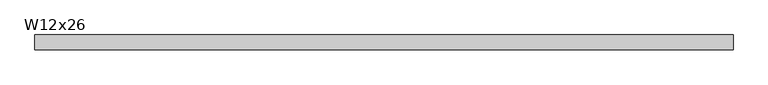
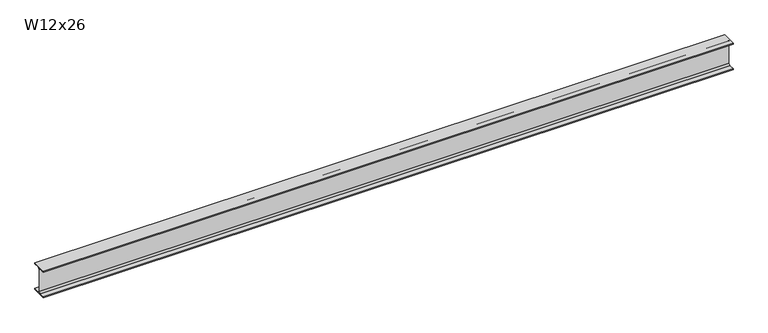
"""IFC4 building model written with IfcOpenShell, lengths in millimetres: beam geometry, RME W-Wide Flange : W12x26."""

from ifc_helpers import new_model, si_unit, point, frame, frame_2d, origin, place, context, project, spatial, polyline, circle_curve, trimmed, segment, composite_curve, outline, extrude, source, transform, mapped, element, save


def w12x26_92753f13(model_context):
    return source(origin(), model_context, "Body", "SweptSolid", [
        extrude(outline(composite_curve([segment(polyline([(82.423, -145.288), (82.423, -154.94), (-82.423, -154.94), (-82.423, -145.288), (-20.2565, -145.288)]), True, "CONTINUOUS"), segment(trimmed(circle_curve(frame_2d((-20.2565, -127.9525)), 17.3355), [point((-20.2565, -145.288))], [point((-2.921, -127.9525))], True, "CARTESIAN"), True, "CONTINUOUS"), segment(polyline([(-2.921, -127.9525), (-2.921, 127.9525)]), True, "CONTINUOUS"), segment(trimmed(circle_curve(frame_2d((-20.2565, 127.9525)), 17.3355), [point((-2.921, 127.9525))], [point((-20.2565, 145.288))], True, "CARTESIAN"), True, "CONTINUOUS"), segment(polyline([(-20.2565, 145.288), (-82.423, 145.288), (-82.423, 154.94), (82.423, 154.94), (82.423, 145.288), (20.2565, 145.288)]), True, "CONTINUOUS"), segment(trimmed(circle_curve(frame_2d((20.2565, 127.9525)), 17.3355), [point((20.2565, 145.288))], [point((2.921, 127.9525))], True, "CARTESIAN"), True, "CONTINUOUS"), segment(polyline([(2.921, 127.9525), (2.921, -127.9525)]), True, "CONTINUOUS"), segment(trimmed(circle_curve(frame_2d((20.2565, -127.9525)), 17.3355), [point((2.921, -127.9525))], [point((20.2565, -145.288))], True, "CARTESIAN"), True, "CONTINUOUS"), segment(polyline([(20.2565, -145.288), (82.423, -145.288)]), True, "CONTINUOUS")], self_intersect=False)), frame((-3823.589, 0.0, 0.0), z_axis=(1.0, 0.0, 0.0), x_axis=(0.0, 1.0, 0.0)), (0.0, 0.0, 1.0), 7664.831),
    ])


if __name__ == "__main__":
    model = new_model("IFC4")
    model_context = context("Model", 3, world=origin())
    ifc_project = project(units=[si_unit("LENGTHUNIT", "METRE", prefix="MILLI")], contexts=[model_context])
    site = spatial("IfcSite", under=ifc_project)
    building = spatial("IfcBuilding", under=site)
    placement = place(None, origin())
    w12x26_shape = w12x26_92753f13(model_context)
    element("IfcBeam", 1, ObjectType="RME W-Wide Flange : W12x26", at=placement, inside=building, context=model_context, shape_type="MappedRepresentation", body=[
        mapped(w12x26_shape, transform((0.0, 0.0, 0.0), x_axis=(1.0, 0.0, 0.0), y_axis=(0.0, 1.0, 0.0), z_axis=(0.0, 0.0, 1.0))),
    ])
    save(model, "model.ifc")

# Revit data of these elements
# Type "RME W-Wide Flange : W12x26"
#   WELD P [instance default] = ""
#   WELD LE [instance default] = ""
#   WELD D [instance default] = ""
#   TOP SECTION SIZE [instance default] = ""
#   TOP SECTION LENGTH [instance default] = ""
#   REMARKS [instance default] = ""
#   REINF TYPE [instance default] = ""
#   Nominal Size = "W24"
#   End Bearing Capacity [instance default] = ""
#   BOT SECTION SIZE [instance default] = ""
#   BOT SECTION LENGTH [instance default] = ""
#   Assembly Code = "B10"
#   W = 26
#   Start Extension Calculation [instance default] = 10' - 0"
#   Start Extension [instance default] = -0' - 0 1/2"
#   End Extension Calculation [instance default] = 10' - 0"
#   End Extension [instance default] = -0' - 0 1/2"
#   Length [instance default] = 5' - 0"
#   bf = 0' - 6.49"
#   d = 1' - 0.2"
#   k = 0' - 1 1/16"
#   k2 = 0' - 0.6825"
#   tf = 0' - 0.38"
#   tw = 0' - 0.23"
#   A = 0.053125 SF
#   Structural Material [instance default] = Metal - Steel - ASTM A992
# Element 1 (IfcBeam, "RME W-Wide Flange : W12x26")
#   Length = 25' - 10"
#   Materials on its faces: "Metal - Steel - ASTM A992"
# Materials
#   "Metal - Steel - ASTM A992": class "Metal", colour RGB 255 128 0, transparency 0
